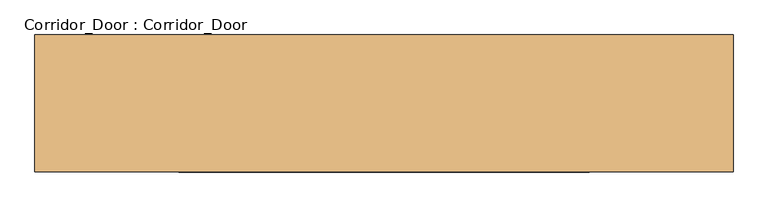
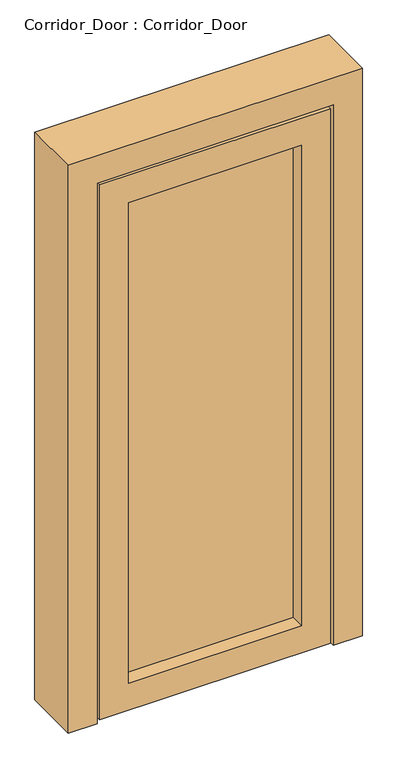
"""IFC4 building model written with IfcOpenShell, lengths in millimetres: door geometry, Corridor_Door : Corridor_Door."""

from ifc_helpers import new_model, si_unit, frame, origin, place, context, project, spatial, polyline, outline, extrude, source, transform, mapped, element, save


def corridor_door_corridor_door_22811d5d(model_context):
    return source(origin(), model_context, "Body", "SweptSolid", [
        extrude(outline(polyline([(525.0, 3485.0), (1125.0, 3485.0), (1125.0, 3475.0), (525.0, 3475.0), (525.0, 3485.0)])), frame((0.0, 0.0, 360.0), z_axis=(0.0, 0.0, 1.0), x_axis=(1.0, 0.0, 0.0)), (0.0, 0.0, 1.0), 1760.0),
        extrude(outline(polyline([(260.0, 1225.0), (2220.0, 1225.0), (2220.0, 425.0), (260.0, 425.0), (260.0, 1225.0)]), holes=[polyline([(360.0, 525.0), (2120.0, 525.0), (2120.0, 1125.0), (360.0, 1125.0), (360.0, 525.0)])]), frame((0.0, 3425.0, 0.0), z_axis=(0.0, 1.0, 0.0), x_axis=(0.0, 0.0, 1.0)), (0.0, 0.0, 1.0), 100.0),
        extrude(outline(polyline([(250.0, 315.0), (250.0, 415.0), (2230.0, 415.0), (2230.0, 1235.0), (250.0, 1235.0), (250.0, 1335.0), (2330.0, 1335.0), (2330.0, 315.0), (250.0, 315.0)])), frame((0.0, 3425.0, 0.0), z_axis=(0.0, 1.0, 0.0), x_axis=(0.0, 0.0, 1.0)), (0.0, 0.0, 1.0), 200.0),
    ])


if __name__ == "__main__":
    model = new_model("IFC4")
    model_context = context("Model", 3, world=origin())
    ifc_project = project(units=[si_unit("LENGTHUNIT", "METRE", prefix="MILLI")], contexts=[model_context])
    site = spatial("IfcSite", under=ifc_project)
    building = spatial("IfcBuilding", under=site)
    placement = place(None, origin())
    corridor_door_corridor_door_shape = corridor_door_corridor_door_22811d5d(model_context)
    element("IfcDoor", 1, ObjectType="Corridor_Door : Corridor_Door", at=placement, inside=building, context=model_context, shape_type="MappedRepresentation", body=[
        mapped(corridor_door_corridor_door_shape, transform((0.0, 0.0, 0.0), x_axis=(1.0, 0.0, 0.0), y_axis=(0.0, 1.0, 0.0), z_axis=(0.0, 0.0, 1.0))),
    ])
    save(model, "model.ifc")

# Revit data of these elements
# Type "Corridor_Door : Corridor_Door"
#   Type Mark = "50"
#   NameOverride = "Corridor_Door"
# Element 1 (IfcDoor, "Corridor_Door : Corridor_Door")
#   Materials on its faces: "IfcSurfaceStyle #392", "IfcSurfaceStyle #398"
# Materials
#   "IfcSurfaceStyle #392": class "Unassigned", colour RGB 204 204 204, transparency 0
#   "IfcSurfaceStyle #398": class "Unassigned", colour RGB 93 183 203, transparency 0.85
